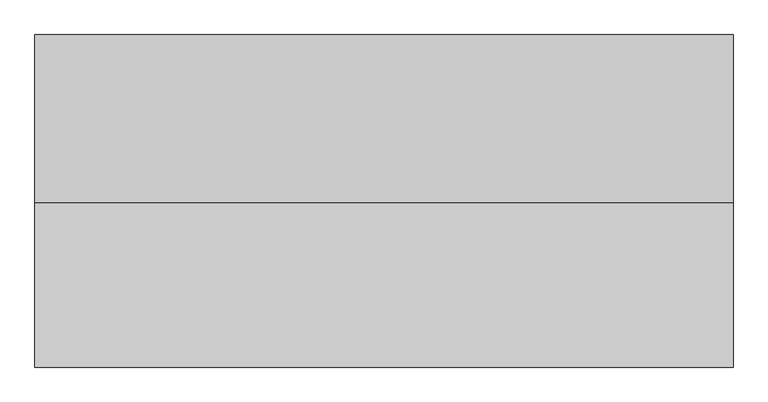
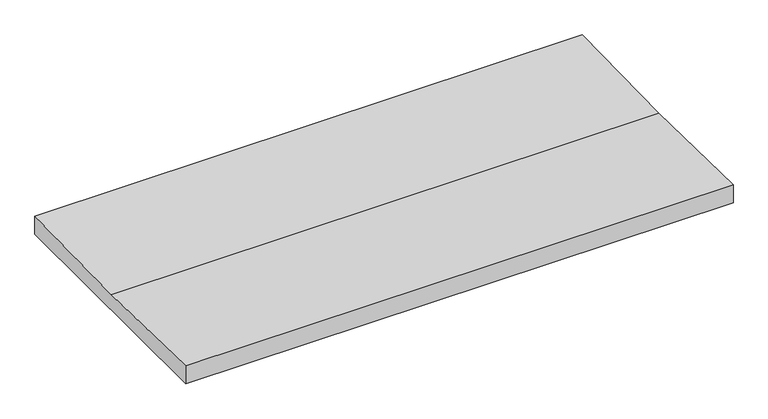
"""IFC4 building model written with IfcOpenShell, lengths in millimetres: proxy geometry, FIRESTONE INSULATION1 : FIRESTONE INSULATION001."""

from ifc_helpers import new_model, si_unit, frame, origin, place, context, project, spatial, polyline, outline, extrude, source, transform, mapped, element, save


def generic_models_233e500c(model_context):
    return source(origin(), model_context, "Body", "SweptSolid", [
        extrude(outline(polyline([(-5343.2581759, 40201.5164062), (-4872.9612169, 40191.7185529), (-4390.315464, 40201.5164062), (-4390.315464, 40131.746), (-5343.2581759, 40131.746), (-5343.2581759, 40201.5164062)])), frame((12382.7678845, 0.0, 0.0), z_axis=(1.0, 0.0, 0.0), x_axis=(0.0, 1.0, 0.0)), (0.0, 0.0, 1.0), 2000.25),
    ])


if __name__ == "__main__":
    model = new_model("IFC4")
    model_context = context("Model", 3, world=origin())
    ifc_project = project(units=[si_unit("LENGTHUNIT", "METRE", prefix="MILLI")], contexts=[model_context])
    site = spatial("IfcSite", under=ifc_project)
    building = spatial("IfcBuilding", under=site)
    placement = place(None, origin())
    generic_models_shape = generic_models_233e500c(model_context)
    element("IfcBuildingElementProxy", 1, Name="FIRESTONE INSULATION1 : FIRESTONE INSULATION001", ObjectType="FIRESTONE INSULATION1 : FIRESTONE INSULATION001", at=placement, inside=building, context=model_context, shape_type="MappedRepresentation", body=[
        mapped(generic_models_shape, transform((0.0, 0.0, 0.0), x_axis=(1.0, 0.0, 0.0), y_axis=(0.0, 1.0, 0.0), z_axis=(0.0, 0.0, 1.0))),
    ])
    save(model, "model.ifc")

# Revit data of these elements
# Type "FIRESTONE INSULATION1 : FIRESTONE INSULATION001"
#   NameOverride = "FIRESTONE INSULATION001"
# Element 1 (IfcBuildingElementProxy, "FIRESTONE INSULATION1 : FIRESTONE INSULATION001")
#   Materials on its faces: "TAPERED 2X SLEEPERS - SLOPED TO DRAIN"
# Materials
#   "TAPERED 2X SLEEPERS - SLOPED TO DRAIN": class "Unassigned", colour RGB 234 198 178, transparency 0
